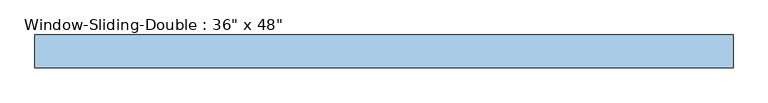
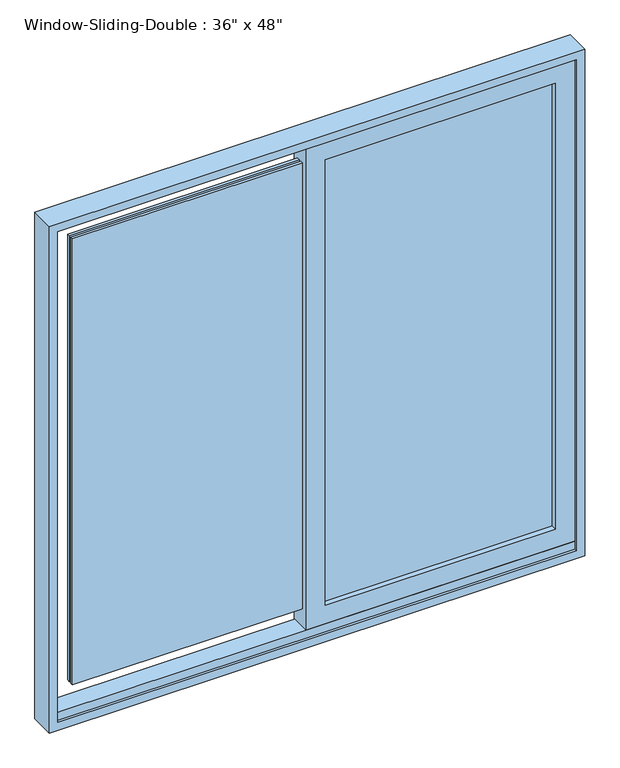
"""IFC4 building model written with IfcOpenShell, lengths in millimetres: window geometry."""

from ifc_helpers import new_model, si_unit, frame, origin, place, context, project, spatial, polyline, outline, extrude, faceted_brep, source, transform, mapped, element, save


def window_8fd24714(model_context):
    return source(origin(), model_context, "Body", "SolidModel", [
        faceted_brep([(-609.6, -10.16, 914.4), (-609.6, 46.99, 914.4), (609.6, 46.99, 914.4), (609.6, -10.16, 914.4), (-568.6778905, 46.99, 2092.6778905), (-568.6778905, 40.64, 2092.6778905), (-568.6778905, 40.64, 952.5), (-568.6778905, 40.64, 933.45), (-568.6778905, 46.99, 933.45), (568.6778905, 40.64, 2092.6778905), (568.6778905, 40.64, 952.5), (590.55, 40.64, 952.5), (590.55, 40.64, 2114.55), (-590.55, 40.64, 2114.55), (-590.55, 40.64, 952.5), (-590.55, -10.16, 2114.55), (-590.55, -10.16, 933.45), (-590.55, -3.81, 933.45), (-590.55, -3.81, 952.5), (609.6, -10.16, 2133.6), (-609.6, -10.16, 2133.6), (590.55, -10.16, 2114.55), (590.55, -10.16, 933.45), (-609.6, 46.99, 2133.6), (609.6, 46.99, 2133.6), (568.6778905, 46.99, 933.45), (568.6778905, 46.99, 2092.6778905), (568.6778905, 40.64, 933.45), (590.55, -3.81, 952.5), (590.55, -3.81, 933.45)], [[[0, 1, 2, 3]], [[4, 5, 6, 7, 8]], [[5, 9, 10, 11, 12, 13, 14, 6]], [[13, 15, 16, 17, 18, 14]], [[0, 3, 19, 20], [21, 22, 16, 15]], [[23, 1, 0, 20]], [[2, 1, 23, 24], [4, 8, 25, 26]], [[5, 4, 26, 9]], [[13, 12, 21, 15]], [[20, 19, 24, 23]], [[9, 26, 25, 27, 10]], [[21, 12, 11, 28, 29, 22]], [[19, 3, 2, 24]], [[7, 27, 25, 8]], [[27, 7, 6, 10]], [[10, 6, 14, 18, 28, 11]], [[28, 18, 17, 29]], [[16, 22, 29, 17]]]),
        extrude(outline(polyline([(546.1, 27.94), (546.1, 21.59), (22.225, 21.59), (22.225, 27.94), (546.1, 27.94)])), frame((0.0, 0.0, 996.95), z_axis=(0.0, 0.0, 1.0), x_axis=(1.0, 0.0, 0.0)), (0.0, 0.0, 1.0), 1073.15),
        extrude(outline(polyline([(546.1, 15.24), (546.1, 8.89), (22.225, 8.89), (22.225, 15.24), (546.1, 15.24)])), frame((0.0, 0.0, 996.95), z_axis=(0.0, 0.0, 1.0), x_axis=(1.0, 0.0, 0.0)), (0.0, 0.0, 1.0), 1073.15),
        extrude(outline(polyline([(-22.225, 27.94), (-22.225, 21.59), (-546.1, 21.59), (-546.1, 27.94), (-22.225, 27.94)])), frame((0.0, 0.0, 996.95), z_axis=(0.0, 0.0, 1.0), x_axis=(1.0, 0.0, 0.0)), (0.0, 0.0, 1.0), 1073.15),
        extrude(outline(polyline([(-22.225, 15.24), (-22.225, 8.89), (-546.1, 8.89), (-546.1, 15.24), (-22.225, 15.24)])), frame((0.0, 0.0, 996.95), z_axis=(0.0, 0.0, 1.0), x_axis=(1.0, 0.0, 0.0)), (0.0, 0.0, 1.0), 1073.15),
        extrude(outline(polyline([(952.5, 590.55), (2114.55, 590.55), (2114.55, -22.225), (952.5, -22.225), (952.5, 590.55)]), holes=[polyline([(996.95, 22.225), (2070.1, 22.225), (2070.1, 546.1), (996.95, 546.1), (996.95, 22.225)])]), frame((0.0, -3.81, 0.0), z_axis=(0.0, 1.0, 0.0), x_axis=(0.0, 0.0, 1.0)), (0.0, 0.0, 1.0), 44.45),
    ])


if __name__ == "__main__":
    model = new_model("IFC4")
    model_context = context("Model", 3, world=origin())
    ifc_project = project(units=[si_unit("LENGTHUNIT", "METRE", prefix="MILLI")], contexts=[model_context])
    site = spatial("IfcSite", under=ifc_project)
    building = spatial("IfcBuilding", under=site)
    placement = place(None, origin())
    window_shape = window_8fd24714(model_context)
    element("IfcWindow", 1, ObjectType="Window-Sliding-Double : 36\" x 48\"", at=placement, inside=building, context=model_context, shape_type="MappedRepresentation", body=[
        mapped(window_shape, transform((0.0, 0.0, 0.0), x_axis=(1.0, 0.0, 0.0), y_axis=(0.0, 1.0, 0.0), z_axis=(0.0, 0.0, 1.0))),
    ])
    save(model, "model.ifc")

# Revit data of these elements
# Type "Window-Sliding-Double : 36\" x 48\""
#   Type Mark = "24"
#   Fire Rating = "0.5h"
#   Assembly Code = "B2020100"
#   Analytic Construction = "Double glazing - domestic"
#   Window Inset [instance default] = 0' - 0"
#   Wall Thickness [instance default] = 0' - 6"
#   Visual Light Transmittance = 0.81
#   Thermal Resistance (R) = 1.8146 (h·ft²·°F)/BTU
#   Solar Heat Gain Coefficient = 0.76
#   Muntin Width = 1' - 8 5/8"
#   Muntin Height = 3' - 6 1/4"
#   Interior Wall Closure [instance default] = 0' - 2 3/4"
#   Heat Transfer Coefficient (U) = 0.5511 BTU/(h·ft²·°F)
#   Frame Extension [instance default] = 0' - 0 1/4"
#   Exterior Wall Closure [instance default] = 0' - 1 1/4"
#   Rough Width = 4' - 0 1/2"
#   Rough Height = 4' - 0 1/2"
#   Height = 4' - 0"
#   Extension Jamb [instance default] = 0' - 2 3/4"
#   Default Sill Height = 3' - 0"
#   Width = 4' - 0"
#   Interior Trim Visibility [instance default] = yes
#   Indicator Visibility [instance default] = yes
#   Exterior Trim Visibility [instance default] = yes
#   Muntin Visibility = yes
#   Extension Jamb Visibility [instance default] = yes
#   Muntin Pattern = Muntin Pattern_2x2 : Muntin Pattern_2x2
#   Interior Trim Material = Wood - Stained
#   Interior Trim = Trim-Window-Interior-Flat : Picture Frame
#   Interior Frame Material = Wood - Stained
#   Glass Panel Material = Glass
#   Exterior Trim Material = Clad - White
#   Exterior Trim = Trim-Window-Exterior-Flat : with Sill
#   Exterior Frame Material = Clad - White
#   Wall Closure = (empty or 0)
# Element 1 (IfcWindow, "Window-Sliding-Double : 36\" x 48\"")
#   Wall Thickness = 0' - 2 1/2"
#   Extension Jamb = 0' - 1"
#   Extension Jamb Visibility = no
#   Materials on its faces: "Glass", "Wood - Stained", "Clad - White"
# Materials
#   "Wood - Stained": class "Wood", colour RGB 224 178 126, transparency 0, Cost = 0
#   "Glass": class "Glass", colour RGB 0 128 192, transparency 0.75, Description = "Soda Lime Glass", Cost = 0
#   "Clad - White": class "Wood", colour RGB 242 242 238, transparency 0, Cost = 0
